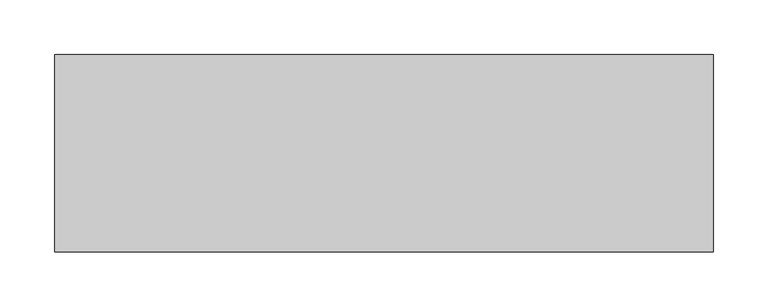
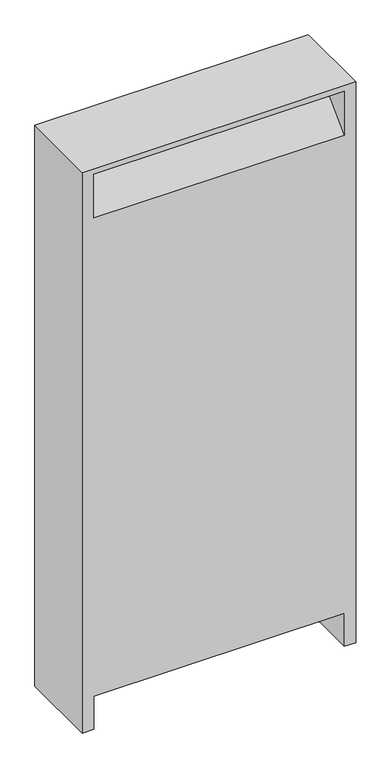
"""IFC4 building model written with IfcOpenShell, lengths in millimetres: proxy geometry, Dry Type Transformer - 480-208Y120 - NEMA Type 2 : Small Power Dist Board."""

import ifcopenshell
import ifcopenshell.guid

model = None  # the IFC model being written
_history = None  # IfcOwnerHistory: only IFC2X3 demands one
_inside = {}  # id of a spatial element -> (the spatial element, [elements in it])
_under = {}  # id of a project, library or spatial element -> (it, [spatial elements below it])
_declared = {}  # id of a project -> (the project, [libraries it declares])
_typed = {}  # id of a type object -> (the type object, [elements of that type])
_made_of = {}  # id of a material, layer set ... -> (it, [elements and type objects made of it])


def new_model(schema):
    """Start an empty IFC model of exactly this schema.

    Asked for "IFC4X3", IfcOpenShell would pick the latest addendum, in which some entities
    have other attributes; the version numbers below select the first issue.
    IFC2X3 requires an IfcOwnerHistory on every rooted entity: one is made here for all.
    """
    global model, _history
    if schema == "IFC4X3":
        model = ifcopenshell.file(schema_version=(4, 3, 0, 0))
    else:
        model = ifcopenshell.file(schema=schema)
    _inside.clear()
    _under.clear()
    _declared.clear()
    _typed.clear()
    _made_of.clear()
    _history = None
    if model.schema == "IFC2X3":
        org = make("IfcOrganization", Name="unknown")
        user = make(
            "IfcPersonAndOrganization",
            ThePerson=make("IfcPerson", FamilyName="unknown"),
            TheOrganization=org,
        )
        app = make(
            "IfcApplication",
            ApplicationDeveloper=org,
            Version="unknown",
            ApplicationFullName="unknown",
            ApplicationIdentifier="unknown",
        )
        _history = make(
            "IfcOwnerHistory",
            OwningUser=user,
            OwningApplication=app,
            ChangeAction="ADDED",
            CreationDate=0,
        )
    return model


def make(cls, **values):
    """One entity of the class cls with the attributes given. An attribute that is None is left unset."""
    return model.create_entity(
        cls, **{name: value for name, value in values.items() if value is not None}
    )


def rooted(cls, **values):
    """An entity with a GlobalId (a new one), such as an element, a storey or a relation."""
    return make(cls, GlobalId=ifcopenshell.guid.new(), OwnerHistory=_history, **values)


def si_unit(unit_type, name, prefix=None):
    """IfcSIUnit, for example si_unit("LENGTHUNIT", "METRE", prefix="MILLI")."""
    return make("IfcSIUnit", UnitType=unit_type, Prefix=prefix, Name=name)


def assignment(units):
    """IfcUnitAssignment: the units of a project."""
    return None if units is None else make("IfcUnitAssignment", Units=units)


def point(xyz):
    """IfcCartesianPoint."""
    return None if xyz is None else make("IfcCartesianPoint", Coordinates=xyz)


def direction(xyz):
    """IfcDirection."""
    return None if xyz is None else make("IfcDirection", DirectionRatios=xyz)


def frame(location, z_axis=None, x_axis=None):
    """IfcAxis2Placement3D, a coordinate frame: its origin and axes. An axis left out is left unset."""
    return make(
        "IfcAxis2Placement3D",
        Location=point(location),
        Axis=direction(z_axis),
        RefDirection=direction(x_axis),
    )


def origin():
    """The frame at (0, 0, 0) with its axes left unset."""
    return frame((0.0, 0.0, 0.0))


def place(relative_to, where):
    """IfcLocalPlacement: puts the frame where relative to a parent placement (None: the world)."""
    return make(
        "IfcLocalPlacement", PlacementRelTo=relative_to, RelativePlacement=where
    )


def context(
    kind, dimensions, precision=None, world=None, true_north=None, identifier=None
):
    """IfcGeometricRepresentationContext, for example the 3D "Model" context."""
    return make(
        "IfcGeometricRepresentationContext",
        ContextIdentifier=identifier,
        ContextType=kind,
        CoordinateSpaceDimension=dimensions,
        Precision=precision,
        WorldCoordinateSystem=world,
        TrueNorth=true_north,
    )


def project(units=None, contexts=None):
    """IfcProject with its units and contexts."""
    return rooted(
        "IfcProject",
        Name="project",
        RepresentationContexts=contexts,
        UnitsInContext=assignment(units),
    )


def spatial(cls, under=None, at=None, **own):
    """A site, building, storey or space (cls), placed at a placement, below another one or the project."""
    s = rooted(cls, ObjectPlacement=at, **own)
    if under is not None:
        _under.setdefault(under.id(), (under, []))[1].append(s)
    return s


def faces_of(points, faces, orient=None, outer=None):
    """IfcFace entities. A face is a list of loops; a loop is a list of indices into points, from 0.

    orient and outer hold one flag for each loop. By default every Orientation is true, the
    first loop of a face is its IfcFaceOuterBound and the others are IfcFaceBound.
    """
    made = []
    for i, loops in enumerate(faces):
        bounds = []
        for j, loop in enumerate(loops):
            is_outer = j == 0 if outer is None else outer[i][j]
            bounds.append(
                make(
                    "IfcFaceOuterBound" if is_outer else "IfcFaceBound",
                    Bound=make("IfcPolyLoop", Polygon=[points[k] for k in loop]),
                    Orientation=True if orient is None else orient[i][j],
                )
            )
        made.append(make("IfcFace", Bounds=bounds))
    return made


def faceted_brep(points, faces, orient=None, outer=None, voids=None):
    """IfcFacetedBrep: a solid bounded by flat faces; with voids (closed shells), ...WithVoids."""
    shared = [point(p) for p in points]
    hull = make("IfcClosedShell", CfsFaces=faces_of(shared, faces, orient, outer))
    if voids is None:
        return make("IfcFacetedBrep", Outer=hull)
    return make(
        "IfcFacetedBrepWithVoids",
        Outer=hull,
        Voids=[
            make(cls, CfsFaces=faces_of(shared, fs, o, b)) for cls, fs, o, b in voids
        ],
    )


def shape(context_of_items, identifier, shape_type, items):
    """IfcShapeRepresentation: the items that make up one representation, for example the "Body"."""
    return make(
        "IfcShapeRepresentation",
        ContextOfItems=context_of_items,
        RepresentationIdentifier=identifier,
        RepresentationType=shape_type,
        Items=items,
    )


def source(mapping_origin, context_of_items, identifier, shape_type, items):
    """IfcRepresentationMap: a shape defined once, which mapped items show again and again."""
    return make(
        "IfcRepresentationMap",
        MappingOrigin=mapping_origin,
        MappedRepresentation=shape(context_of_items, identifier, shape_type, items),
    )


def transform(
    local_origin,
    x_axis=None,
    y_axis=None,
    z_axis=None,
    scale=None,
    scale2=None,
    scale3=None,
    uniform=True,
):
    """IfcCartesianTransformationOperator3D, or its non-uniform kind. x_axis, y_axis, z_axis: its Axis1, 2, 3."""
    if uniform:
        return make(
            "IfcCartesianTransformationOperator3D",
            Axis1=direction(x_axis),
            Axis2=direction(y_axis),
            LocalOrigin=point(local_origin),
            Scale=scale,
            Axis3=direction(z_axis),
        )
    return make(
        "IfcCartesianTransformationOperator3DnonUniform",
        Axis1=direction(x_axis),
        Axis2=direction(y_axis),
        LocalOrigin=point(local_origin),
        Scale=scale,
        Axis3=direction(z_axis),
        Scale2=scale2,
        Scale3=scale3,
    )


def mapped(mapping_source, mapping_target):
    """IfcMappedItem: shows the shape of a source again, moved by a transform."""
    return make(
        "IfcMappedItem", MappingSource=mapping_source, MappingTarget=mapping_target
    )


def made_of(thing, what):
    """Note that an element or type object is made of a material, layer set ...; save() writes the relation."""
    if what is not None:
        _made_of.setdefault(what.id(), (what, []))[1].append(thing)
    return thing


def element(
    cls,
    number,
    at=None,
    inside=None,
    cuts=None,
    type_object=None,
    material=None,
    context=None,
    identifier="Body",
    shape_type=None,
    held_by="IfcProductDefinitionShape",
    body=None,
    shapes=None,
    **own,
):
    """One element of the class cls, such as IfcWall. Its Tag is "e" and its number.

    at: its placement. inside: the storey or other place that contains it. cuts: it is an
    opening in that element (IfcRelVoidsElement). A single representation is given by context,
    identifier, shape_type and body (its items); several are given by shapes. held_by: the class
    of the entity that holds the representations. save() writes the other relations.
    """
    e = rooted(cls, Tag="e%d" % number, ObjectPlacement=at, **own)
    if body is not None:
        shapes = [shape(context, identifier, shape_type, body)]
    if shapes is not None:
        e.Representation = make(held_by, Representations=shapes)
    if inside is not None:
        _inside.setdefault(inside.id(), (inside, []))[1].append(e)
    if cuts is not None:
        rooted(
            "IfcRelVoidsElement", RelatingBuildingElement=cuts, RelatedOpeningElement=e
        )
    if type_object is not None:
        _typed.setdefault(type_object.id(), (type_object, []))[1].append(e)
    return made_of(e, material)


def aggregate(whole, parts):
    """IfcRelAggregates: a whole, such as a stair, and the parts it consists of."""
    return rooted("IfcRelAggregates", RelatingObject=whole, RelatedObjects=parts)


def save(model, path):
    """Write the relations noted so far, then the file.

    IfcRelAggregates (storeys below a building ...), IfcRelContainedInSpatialStructure (elements
    in a storey), IfcRelDefinesByType, IfcRelAssociatesMaterial and IfcRelDeclares: one each for
    every whole, place, type object, material and project.
    """
    for whole, parts in _under.values():
        aggregate(whole, parts)
    for where, things in _inside.values():
        rooted(
            "IfcRelContainedInSpatialStructure",
            RelatedElements=things,
            RelatingStructure=where,
        )
    for kind, things in _typed.values():
        rooted("IfcRelDefinesByType", RelatedObjects=things, RelatingType=kind)
    for what, things in _made_of.values():
        rooted("IfcRelAssociatesMaterial", RelatedObjects=things, RelatingMaterial=what)
    for by, libraries in _declared.values():
        rooted("IfcRelDeclares", RelatingContext=by, RelatedDefinitions=libraries)
    model.write(path)


def electrical_equipment_ed7dd24e(model_context):
    return source(origin(), model_context, "Body", "Brep", [
        faceted_brep([(300.0, 204.7158651, 1300.0), (300.0, 384.7158651, 1300.0), (-300.0, 384.7158651, 1300.0), (-300.0, 204.7158651, 1300.0), (-300.0, 204.7158651, 0.0), (-300.0, 384.7158651, 0.0), (-274.6, 384.7158651, 0.0), (-274.6, 204.7158651, 0.0), (300.0, 384.7158651, 0.0), (300.0, 204.7158651, 0.0), (274.6, 204.7158651, 0.0), (274.6, 384.7158651, 0.0), (274.6, 384.7158651, 76.2), (-274.6, 384.7158651, 76.2), (274.6, 384.7158651, 1185.7), (274.6, 384.7158651, 1287.3), (-274.6, 384.7158651, 1287.3), (-274.6, 384.7158651, 1185.7), (-274.6, 204.7158651, 76.2), (274.6, 204.7158651, 76.2), (274.6, 204.7158651, 1287.3), (274.6, 204.7158651, 1185.7), (-274.6, 204.7158651, 1185.7), (-274.6, 204.7158651, 1287.3), (274.6, 294.7158651, 1275.7), (-274.6, 294.7158651, 1275.7)], [[[0, 1, 2, 3]], [[4, 5, 6, 7]], [[8, 9, 10, 11]], [[1, 0, 9, 8]], [[2, 1, 8, 11, 12, 13, 6, 5], [14, 15, 16, 17]], [[3, 2, 5, 4]], [[0, 3, 4, 7, 18, 19, 10, 9], [20, 21, 22, 23]], [[18, 13, 12, 19]], [[13, 18, 7, 6]], [[19, 12, 11, 10]], [[21, 20, 15, 14, 24]], [[23, 22, 25, 17, 16]], [[15, 20, 23, 16]], [[22, 21, 24, 25]], [[24, 14, 17, 25]]]),
    ])


if __name__ == "__main__":
    model = new_model("IFC4")
    model_context = context("Model", 3, world=origin())
    ifc_project = project(units=[si_unit("LENGTHUNIT", "METRE", prefix="MILLI")], contexts=[model_context])
    site = spatial("IfcSite", under=ifc_project)
    building = spatial("IfcBuilding", under=site)
    placement = place(None, origin())
    electrical_equipment_shape = electrical_equipment_ed7dd24e(model_context)
    element("IfcBuildingElementProxy", 1, Name="Dry Type Transformer - 480-208Y120 - NEMA Type 2 : Small Power Dist Board", ObjectType="Dry Type Transformer - 480-208Y120 - NEMA Type 2 : Small Power Dist Board", at=placement, inside=building, context=model_context, shape_type="MappedRepresentation", body=[
        mapped(electrical_equipment_shape, transform((0.0, 0.0, 0.0), x_axis=(1.0, 0.0, 0.0), y_axis=(0.0, 1.0, 0.0), z_axis=(0.0, 0.0, 1.0))),
    ])
    save(model, "model.ifc")

# Revit data of these elements
# Type "Dry Type Transformer - 480-208Y120 - NEMA Type 2 : Small Power Dist Board"
#   built-in parameter 1140083 [instance default] = "Type 2"
#   Transformer Length = 600 mm
#   Primary Voltage = 480 V
#   Transformer Height = 1300 mm
#   built-in parameter 1140140 [instance default] = 1 (stored number, unit not read)
#   Transformer Width = 180 mm
#   built-in parameter 1140142 [instance default] = -1
#   Primary Number of Poles = 3
#   built-in parameter 1140079 [instance default] = 3
#   Transformer Material = none
#   Load Classification = Transformer
#   Default Elevation = 0
#   Assembly Code = ""
#   built-in parameter 1140087 [instance default] = 1
